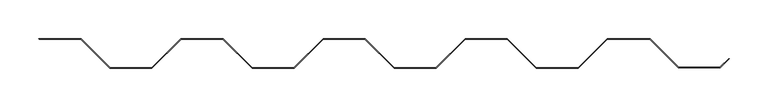
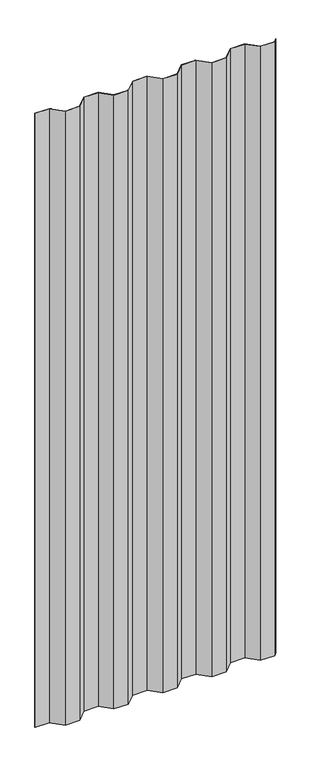
"""IFC4 building model written with IfcOpenShell, lengths in millimetres: proxy geometry, MBCI 7.2-V Panel24 : MBCI 7.2-V Panel-1."""

import ifcopenshell
import ifcopenshell.guid

model = None  # the IFC model being written
_history = None  # IfcOwnerHistory: only IFC2X3 demands one
_inside = {}  # id of a spatial element -> (the spatial element, [elements in it])
_under = {}  # id of a project, library or spatial element -> (it, [spatial elements below it])
_declared = {}  # id of a project -> (the project, [libraries it declares])
_typed = {}  # id of a type object -> (the type object, [elements of that type])
_made_of = {}  # id of a material, layer set ... -> (it, [elements and type objects made of it])


def new_model(schema):
    """Start an empty IFC model of exactly this schema.

    Asked for "IFC4X3", IfcOpenShell would pick the latest addendum, in which some entities
    have other attributes; the version numbers below select the first issue.
    IFC2X3 requires an IfcOwnerHistory on every rooted entity: one is made here for all.
    """
    global model, _history
    if schema == "IFC4X3":
        model = ifcopenshell.file(schema_version=(4, 3, 0, 0))
    else:
        model = ifcopenshell.file(schema=schema)
    _inside.clear()
    _under.clear()
    _declared.clear()
    _typed.clear()
    _made_of.clear()
    _history = None
    if model.schema == "IFC2X3":
        org = make("IfcOrganization", Name="unknown")
        user = make(
            "IfcPersonAndOrganization",
            ThePerson=make("IfcPerson", FamilyName="unknown"),
            TheOrganization=org,
        )
        app = make(
            "IfcApplication",
            ApplicationDeveloper=org,
            Version="unknown",
            ApplicationFullName="unknown",
            ApplicationIdentifier="unknown",
        )
        _history = make(
            "IfcOwnerHistory",
            OwningUser=user,
            OwningApplication=app,
            ChangeAction="ADDED",
            CreationDate=0,
        )
    return model


def make(cls, **values):
    """One entity of the class cls with the attributes given. An attribute that is None is left unset."""
    return model.create_entity(
        cls, **{name: value for name, value in values.items() if value is not None}
    )


def rooted(cls, **values):
    """An entity with a GlobalId (a new one), such as an element, a storey or a relation."""
    return make(cls, GlobalId=ifcopenshell.guid.new(), OwnerHistory=_history, **values)


def si_unit(unit_type, name, prefix=None):
    """IfcSIUnit, for example si_unit("LENGTHUNIT", "METRE", prefix="MILLI")."""
    return make("IfcSIUnit", UnitType=unit_type, Prefix=prefix, Name=name)


def assignment(units):
    """IfcUnitAssignment: the units of a project."""
    return None if units is None else make("IfcUnitAssignment", Units=units)


def point(xyz):
    """IfcCartesianPoint."""
    return None if xyz is None else make("IfcCartesianPoint", Coordinates=xyz)


def direction(xyz):
    """IfcDirection."""
    return None if xyz is None else make("IfcDirection", DirectionRatios=xyz)


def frame(location, z_axis=None, x_axis=None):
    """IfcAxis2Placement3D, a coordinate frame: its origin and axes. An axis left out is left unset."""
    return make(
        "IfcAxis2Placement3D",
        Location=point(location),
        Axis=direction(z_axis),
        RefDirection=direction(x_axis),
    )


def origin():
    """The frame at (0, 0, 0) with its axes left unset."""
    return frame((0.0, 0.0, 0.0))


def place(relative_to, where):
    """IfcLocalPlacement: puts the frame where relative to a parent placement (None: the world)."""
    return make(
        "IfcLocalPlacement", PlacementRelTo=relative_to, RelativePlacement=where
    )


def context(
    kind, dimensions, precision=None, world=None, true_north=None, identifier=None
):
    """IfcGeometricRepresentationContext, for example the 3D "Model" context."""
    return make(
        "IfcGeometricRepresentationContext",
        ContextIdentifier=identifier,
        ContextType=kind,
        CoordinateSpaceDimension=dimensions,
        Precision=precision,
        WorldCoordinateSystem=world,
        TrueNorth=true_north,
    )


def project(units=None, contexts=None):
    """IfcProject with its units and contexts."""
    return rooted(
        "IfcProject",
        Name="project",
        RepresentationContexts=contexts,
        UnitsInContext=assignment(units),
    )


def spatial(cls, under=None, at=None, **own):
    """A site, building, storey or space (cls), placed at a placement, below another one or the project."""
    s = rooted(cls, ObjectPlacement=at, **own)
    if under is not None:
        _under.setdefault(under.id(), (under, []))[1].append(s)
    return s


def polyline(points):
    """IfcPolyline through the points."""
    return make("IfcPolyline", Points=[point(p) for p in points])


def outline(outer, holes=None, kind="AREA"):
    """IfcArbitraryClosedProfileDef: a profile drawn as a closed curve; with holes, ...WithVoids."""
    if holes is None:
        return make("IfcArbitraryClosedProfileDef", ProfileType=kind, OuterCurve=outer)
    return make(
        "IfcArbitraryProfileDefWithVoids",
        ProfileType=kind,
        OuterCurve=outer,
        InnerCurves=holes,
    )


def extrude(swept, where, along, depth):
    """IfcExtrudedAreaSolid: the profile swept, set in the frame where, extruded along a direction by depth."""
    return make(
        "IfcExtrudedAreaSolid",
        SweptArea=swept,
        Position=where,
        ExtrudedDirection=direction(along),
        Depth=depth,
    )


def shape(context_of_items, identifier, shape_type, items):
    """IfcShapeRepresentation: the items that make up one representation, for example the "Body"."""
    return make(
        "IfcShapeRepresentation",
        ContextOfItems=context_of_items,
        RepresentationIdentifier=identifier,
        RepresentationType=shape_type,
        Items=items,
    )


def source(mapping_origin, context_of_items, identifier, shape_type, items):
    """IfcRepresentationMap: a shape defined once, which mapped items show again and again."""
    return make(
        "IfcRepresentationMap",
        MappingOrigin=mapping_origin,
        MappedRepresentation=shape(context_of_items, identifier, shape_type, items),
    )


def transform(
    local_origin,
    x_axis=None,
    y_axis=None,
    z_axis=None,
    scale=None,
    scale2=None,
    scale3=None,
    uniform=True,
):
    """IfcCartesianTransformationOperator3D, or its non-uniform kind. x_axis, y_axis, z_axis: its Axis1, 2, 3."""
    if uniform:
        return make(
            "IfcCartesianTransformationOperator3D",
            Axis1=direction(x_axis),
            Axis2=direction(y_axis),
            LocalOrigin=point(local_origin),
            Scale=scale,
            Axis3=direction(z_axis),
        )
    return make(
        "IfcCartesianTransformationOperator3DnonUniform",
        Axis1=direction(x_axis),
        Axis2=direction(y_axis),
        LocalOrigin=point(local_origin),
        Scale=scale,
        Axis3=direction(z_axis),
        Scale2=scale2,
        Scale3=scale3,
    )


def mapped(mapping_source, mapping_target):
    """IfcMappedItem: shows the shape of a source again, moved by a transform."""
    return make(
        "IfcMappedItem", MappingSource=mapping_source, MappingTarget=mapping_target
    )


def made_of(thing, what):
    """Note that an element or type object is made of a material, layer set ...; save() writes the relation."""
    if what is not None:
        _made_of.setdefault(what.id(), (what, []))[1].append(thing)
    return thing


def element(
    cls,
    number,
    at=None,
    inside=None,
    cuts=None,
    type_object=None,
    material=None,
    context=None,
    identifier="Body",
    shape_type=None,
    held_by="IfcProductDefinitionShape",
    body=None,
    shapes=None,
    **own,
):
    """One element of the class cls, such as IfcWall. Its Tag is "e" and its number.

    at: its placement. inside: the storey or other place that contains it. cuts: it is an
    opening in that element (IfcRelVoidsElement). A single representation is given by context,
    identifier, shape_type and body (its items); several are given by shapes. held_by: the class
    of the entity that holds the representations. save() writes the other relations.
    """
    e = rooted(cls, Tag="e%d" % number, ObjectPlacement=at, **own)
    if body is not None:
        shapes = [shape(context, identifier, shape_type, body)]
    if shapes is not None:
        e.Representation = make(held_by, Representations=shapes)
    if inside is not None:
        _inside.setdefault(inside.id(), (inside, []))[1].append(e)
    if cuts is not None:
        rooted(
            "IfcRelVoidsElement", RelatingBuildingElement=cuts, RelatedOpeningElement=e
        )
    if type_object is not None:
        _typed.setdefault(type_object.id(), (type_object, []))[1].append(e)
    return made_of(e, material)


def aggregate(whole, parts):
    """IfcRelAggregates: a whole, such as a stair, and the parts it consists of."""
    return rooted("IfcRelAggregates", RelatingObject=whole, RelatedObjects=parts)


def save(model, path):
    """Write the relations noted so far, then the file.

    IfcRelAggregates (storeys below a building ...), IfcRelContainedInSpatialStructure (elements
    in a storey), IfcRelDefinesByType, IfcRelAssociatesMaterial and IfcRelDeclares: one each for
    every whole, place, type object, material and project.
    """
    for whole, parts in _under.values():
        aggregate(whole, parts)
    for where, things in _inside.values():
        rooted(
            "IfcRelContainedInSpatialStructure",
            RelatedElements=things,
            RelatingStructure=where,
        )
    for kind, things in _typed.values():
        rooted("IfcRelDefinesByType", RelatedObjects=things, RelatingType=kind)
    for what, things in _made_of.values():
        rooted("IfcRelAssociatesMaterial", RelatedObjects=things, RelatingMaterial=what)
    for by, libraries in _declared.values():
        rooted("IfcRelDeclares", RelatingContext=by, RelatedDefinitions=libraries)
    model.write(path)


def generic_models_0e9549c0(model_context):
    return source(origin(), model_context, "Body", "SweptSolid", [
        extrude(outline(polyline([(587418.0082638, -531601.7259841), (587364.5694989, -531601.7259841), (587363.9741864, -531601.1306716), (587418.2548503, -531601.1306716), (587455.7452503, -531638.6210716), (587509.3637864, -531638.6210716), (587546.8541864, -531601.1306716), (587601.1348503, -531601.1306716), (587638.6252503, -531638.6210716), (587692.2437864, -531638.6210716), (587729.7341864, -531601.1306716), (587784.0148503, -531601.1306716), (587821.5052503, -531638.6210716), (587875.1237864, -531638.6210716), (587912.6141864, -531601.1306716), (587966.8948503, -531601.1306716), (588004.3852503, -531638.6210716), (588058.0037864, -531638.6210716), (588095.4941864, -531601.1306716), (588150.6384503, -531601.1306716), (588187.5192503, -531638.0114716), (588240.6073773, -531638.0114716), (588251.7378112, -531626.8810377), (588252.5246865, -531626.9360614), (588240.8539638, -531638.6067841), (588187.2726638, -531638.6067841), (588150.3918638, -531601.7259841), (588095.7407729, -531601.7259841), (588058.2503729, -531639.2163841), (588004.1386638, -531639.2163841), (587966.6482638, -531601.7259841), (587912.8607729, -531601.7259841), (587875.3703729, -531639.2163841), (587821.2586638, -531639.2163841), (587783.7682638, -531601.7259841), (587729.9807729, -531601.7259841), (587692.4903729, -531639.2163841), (587638.3786638, -531639.2163841), (587600.8882638, -531601.7259841), (587547.1007729, -531601.7259841), (587509.6103729, -531639.2163841), (587455.4986638, -531639.2163841), (587418.0082638, -531601.7259841)])), frame((0.0, 0.0, 6.35), z_axis=(0.0, 0.0, 1.0), x_axis=(1.0, 0.0, 0.0)), (0.0, 0.0, 1.0), 2432.05),
    ])


if __name__ == "__main__":
    model = new_model("IFC4")
    model_context = context("Model", 3, world=origin())
    ifc_project = project(units=[si_unit("LENGTHUNIT", "METRE", prefix="MILLI")], contexts=[model_context])
    site = spatial("IfcSite", under=ifc_project)
    building = spatial("IfcBuilding", under=site)
    placement = place(None, origin())
    generic_models_shape = generic_models_0e9549c0(model_context)
    element("IfcBuildingElementProxy", 1, Name="MBCI 7.2-V Panel24 : MBCI 7.2-V Panel-1", ObjectType="MBCI 7.2-V Panel24 : MBCI 7.2-V Panel-1", at=placement, inside=building, context=model_context, shape_type="MappedRepresentation", body=[
        mapped(generic_models_shape, transform((0.0, 0.0, 0.0), x_axis=(1.0, 0.0, 0.0), y_axis=(0.0, 1.0, 0.0), z_axis=(0.0, 0.0, 1.0))),
    ])
    save(model, "model.ifc")

# Revit data of these elements
# Element 1 (IfcBuildingElementProxy, "MBCI 7.2-V Panel24 : MBCI 7.2-V Panel-1")
#   Materials on its faces: "MTL PANEL"
# Materials
#   "MTL PANEL": class "Generic", colour RGB 239 242 240, transparency 0, Cost = 0
